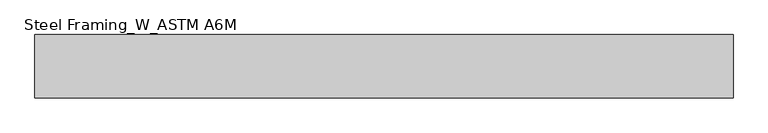
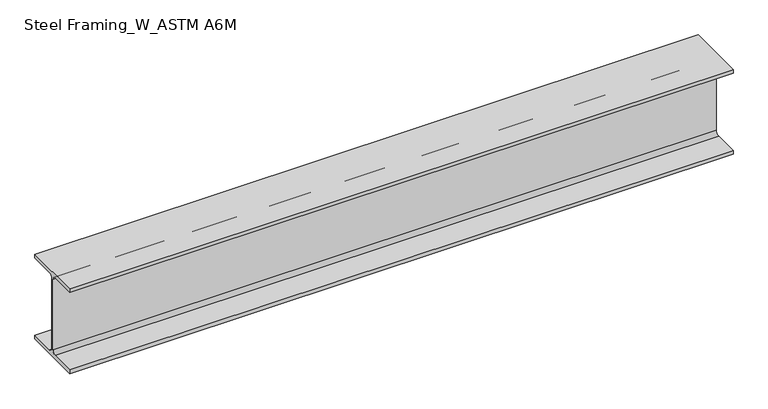
"""IFC4 building model written with IfcOpenShell, lengths in millimetres: beam geometry, Steel Framing_W_ASTM A6M : H_SB_AR_S02_W310x60_B5."""

from ifc_helpers import new_model, si_unit, point, frame, frame_2d, origin, place, context, project, spatial, polyline, circle_curve, trimmed, segment, composite_curve, outline, extrude, source, transform, mapped, element, save


def steel_framing_w_astm_a6m_a97c09f9(model_context):
    return source(origin(), model_context, "Body", "SweptSolid", [
        extrude(outline(composite_curve([segment(polyline([(101.5, -137.9), (101.5, -151.0), (-101.5, -151.0), (-101.5, -137.9), (-16.545, -137.9)]), True, "CONTINUOUS"), segment(trimmed(circle_curve(frame_2d((-16.545, -125.1)), 12.8), [point((-16.545, -137.9))], [point((-3.745, -125.1))], True, "CARTESIAN"), True, "CONTINUOUS"), segment(polyline([(-3.745, -125.1), (-3.745, 125.1)]), True, "CONTINUOUS"), segment(trimmed(circle_curve(frame_2d((-16.545, 125.1)), 12.8), [point((-3.745, 125.1))], [point((-16.545, 137.9))], True, "CARTESIAN"), True, "CONTINUOUS"), segment(polyline([(-16.545, 137.9), (-101.5, 137.9), (-101.5, 151.0), (101.5, 151.0), (101.5, 137.9), (16.545, 137.9)]), True, "CONTINUOUS"), segment(trimmed(circle_curve(frame_2d((16.545, 125.1)), 12.8), [point((16.545, 137.9))], [point((3.745, 125.1))], True, "CARTESIAN"), True, "CONTINUOUS"), segment(polyline([(3.745, 125.1), (3.745, -125.1)]), True, "CONTINUOUS"), segment(trimmed(circle_curve(frame_2d((16.545, -125.1)), 12.8), [point((3.745, -125.1))], [point((16.545, -137.9))], True, "CARTESIAN"), True, "CONTINUOUS"), segment(polyline([(16.545, -137.9), (101.5, -137.9)]), True, "CONTINUOUS")], self_intersect=False)), frame((-1135.3, 0.0, 0.0), z_axis=(1.0, 0.0, 0.0), x_axis=(0.0, 1.0, 0.0)), (0.0, 0.0, 1.0), 2231.6),
    ])


if __name__ == "__main__":
    model = new_model("IFC4")
    model_context = context("Model", 3, world=origin())
    ifc_project = project(units=[si_unit("LENGTHUNIT", "METRE", prefix="MILLI")], contexts=[model_context])
    site = spatial("IfcSite", under=ifc_project)
    building = spatial("IfcBuilding", under=site)
    placement = place(None, origin())
    steel_framing_w_astm_a6m_shape = steel_framing_w_astm_a6m_a97c09f9(model_context)
    element("IfcBeam", 1, ObjectType="Steel Framing_W_ASTM A6M : H_SB_AR_S02_W310x60_B5", at=placement, inside=building, context=model_context, shape_type="MappedRepresentation", body=[
        mapped(steel_framing_w_astm_a6m_shape, transform((0.0, 0.0, 0.0), x_axis=(1.0, 0.0, 0.0), y_axis=(0.0, 1.0, 0.0), z_axis=(0.0, 0.0, 1.0))),
    ])
    save(model, "model.ifc")

# Revit data of these elements
# Type "Steel Framing_W_ASTM A6M : H_SB_AR_S02_W310x60_B5"
#   Type Mark = "B5"
#   Section Name Key = "W12x40"
#   Width = 20.3 cm
#   Web Thickness = 0.749 cm
#   Web Fillet = 1.28 cm
#   Warping Constant = 387000.0 cm⁶
#   Torsional Moment of Inertia = 37.70 cm⁴
#   Section Area = 75.5 cm²
#   Plastic Modulus weak axis = 275.0 cm³
#   Plastic Modulus strong axis = 934.0 cm³
#   Perimeter = 1.38 m²/m
#   Nominal Weight = 60.00 kgf/m
#   Moment of Inertia weak axis = 1840.00 cm⁴
#   Moment of Inertia strong axis = 12800.00 cm⁴
#   Height = 30.2 cm
#   Flange Thickness = 1.31 cm
#   Elastic Modulus weak axis = 180.0 cm³
#   Elastic Modulus strong axis = 844.0 cm³
#   Centroid Vertical = 15.1 cm
#   Centroid Horizontal = 10.15 cm
#   Length [instance default] = 1500 mm
#   Structural Material [instance default] = Steel, 45-345
#   Bolt Spacing = 0
#   Assembly Code = ""
# Element 1 (IfcBeam, "Steel Framing_W_ASTM A6M : H_SB_AR_S02_W310x60_B5")
#   Materials on its faces: "Steel, 45-345"
# Materials
#   "Steel, 45-345": class "Metal", colour RGB 189 187 185, transparency 0, Description = "Steel 345 MPa", Cost = 0
